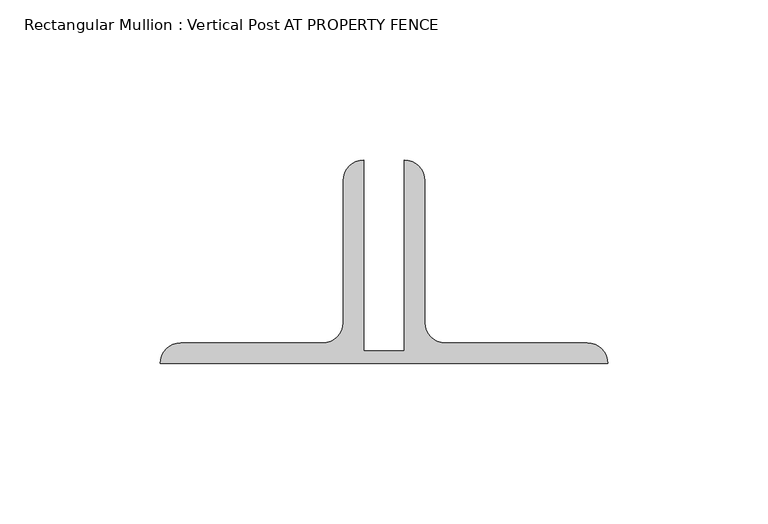
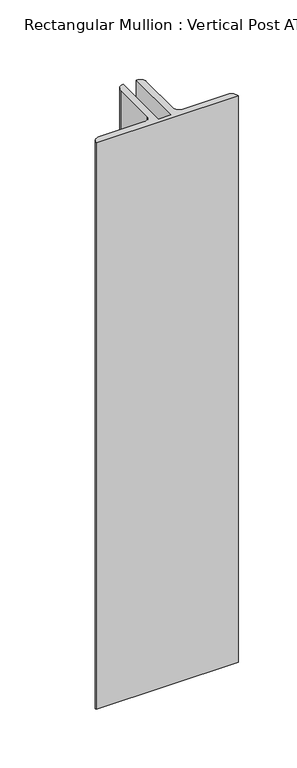
"""IFC4 building model written with IfcOpenShell, lengths in millimetres: member geometry, Rectangular Mullion : Vertical Post AT PROPERTY FENCE."""

from ifc_helpers import new_model, si_unit, point, frame, frame_2d, origin, place, context, project, spatial, polyline, circle_curve, trimmed, segment, composite_curve, outline, extrude, source, transform, mapped, element, save


def rectangular_mullion_vertical_post_at_property_fence_7c31ba12(model_context):
    return source(origin(), model_context, "Body", "SweptSolid", [
        extrude(outline(composite_curve([segment(polyline([(-76.2, 22.9145205), (-63.5, 22.9145205), (-63.5, 82.55)]), True, "CONTINUOUS"), segment(trimmed(circle_curve(frame_2d((-63.5, 76.2)), 6.35), [point((-63.5, 82.55))], [point((-57.15, 76.2))], False, "CARTESIAN"), True, "CONTINUOUS"), segment(polyline([(-57.15, 76.2), (-57.15, 31.75)]), True, "CONTINUOUS"), segment(trimmed(circle_curve(frame_2d((-50.8, 31.75)), 6.35), [point((-57.15, 31.75))], [point((-50.8, 25.4))], True, "CARTESIAN"), True, "CONTINUOUS"), segment(polyline([(-50.8, 25.4), (-6.35, 25.4)]), True, "CONTINUOUS"), segment(trimmed(circle_curve(frame_2d((-6.35, 19.05)), 6.35), [point((-6.35, 25.4))], [point((0.0, 19.05))], False, "CARTESIAN"), True, "CONTINUOUS"), segment(polyline([(0.0, 19.05), (-139.7, 19.05)]), True, "CONTINUOUS"), segment(trimmed(circle_curve(frame_2d((-133.35, 19.05)), 6.35), [point((-139.7, 19.05))], [point((-133.35, 25.4))], False, "CARTESIAN"), True, "CONTINUOUS"), segment(polyline([(-133.35, 25.4), (-88.9, 25.4)]), True, "CONTINUOUS"), segment(trimmed(circle_curve(frame_2d((-88.9, 31.75)), 6.35), [point((-88.9, 25.4))], [point((-82.55, 31.75))], True, "CARTESIAN"), True, "CONTINUOUS"), segment(polyline([(-82.55, 31.75), (-82.55, 76.2)]), True, "CONTINUOUS"), segment(trimmed(circle_curve(frame_2d((-76.2, 76.2)), 6.35), [point((-82.55, 76.2))], [point((-76.2, 82.55))], False, "CARTESIAN"), True, "CONTINUOUS"), segment(polyline([(-76.2, 82.55), (-76.2, 22.9145205)]), True, "CONTINUOUS")], self_intersect=False)), frame((0.0, 0.0, -588.8534967), z_axis=(0.0, 0.0, 1.0), x_axis=(1.0, 0.0, 0.0)), (0.0, 0.0, 1.0), 588.8534967),
    ])


if __name__ == "__main__":
    model = new_model("IFC4")
    model_context = context("Model", 3, world=origin())
    ifc_project = project(units=[si_unit("LENGTHUNIT", "METRE", prefix="MILLI")], contexts=[model_context])
    site = spatial("IfcSite", under=ifc_project)
    building = spatial("IfcBuilding", under=site)
    placement = place(None, origin())
    rectangular_mullion_vertical_post_at_property_fence_shape = rectangular_mullion_vertical_post_at_property_fence_7c31ba12(model_context)
    element("IfcMember", 1, ObjectType="Rectangular Mullion : Vertical Post AT PROPERTY FENCE", at=placement, inside=building, context=model_context, shape_type="MappedRepresentation", body=[
        mapped(rectangular_mullion_vertical_post_at_property_fence_shape, transform((0.0, 0.0, 0.0), x_axis=(1.0, 0.0, 0.0), y_axis=(0.0, 1.0, 0.0), z_axis=(0.0, 0.0, 1.0))),
    ])
    save(model, "model.ifc")

# Revit data of these elements
# Type "Rectangular Mullion : Vertical Post AT PROPERTY FENCE"
#   built-in parameter 1007351 = -0.0625 (stored number, unit not read)
#   built-in parameter 1007322 = 0.0126789 (stored number, unit not read)
#   built-in parameter 1007321 = 0.229167 (stored number, unit not read)
#   built-in parameter 1007320 = 0.229167 (stored number, unit not read)
# Element 1 (IfcMember, "Rectangular Mullion : Vertical Post AT PROPERTY FENCE")
#   Materials on its faces: "MAIN FENCE POST: (2) BACK/BACK GALVANIZED ANGLES (2) L2 1/2 X 2 1/2 X 1/4\") ANCHORED TO 8\"W X 42\" DEEP CONCRETE FOOTING(1)"
# Materials
#   "MAIN FENCE POST: (2) BACK/BACK GALVANIZED ANGLES (2) L2 1/2 X 2 1/2 X 1/4\") ANCHORED TO 8\"W X 42\" DEEP CONCRETE FOOTING(1)": class "Unassigned", colour RGB 211 211 211, transparency 0, Cost = 0
